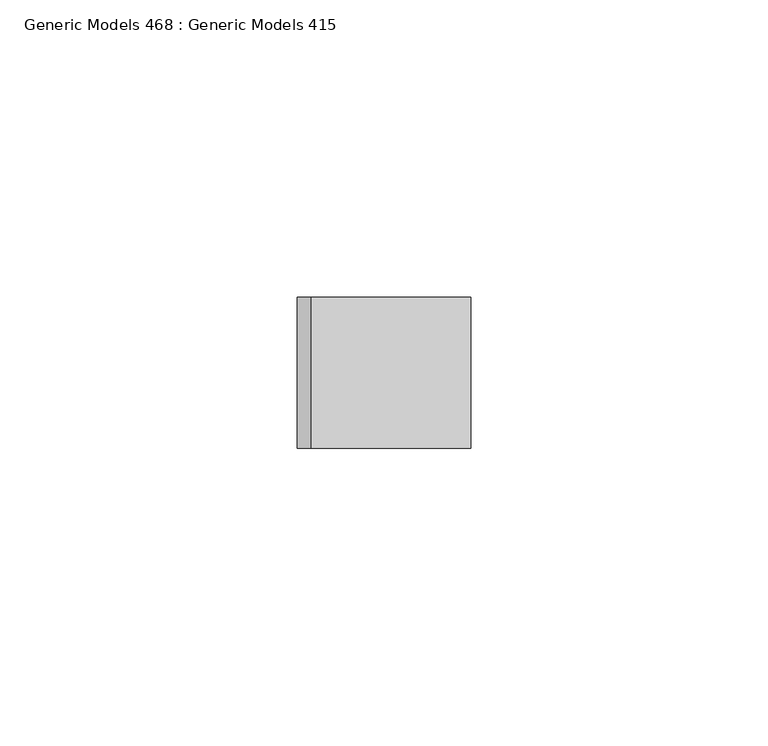
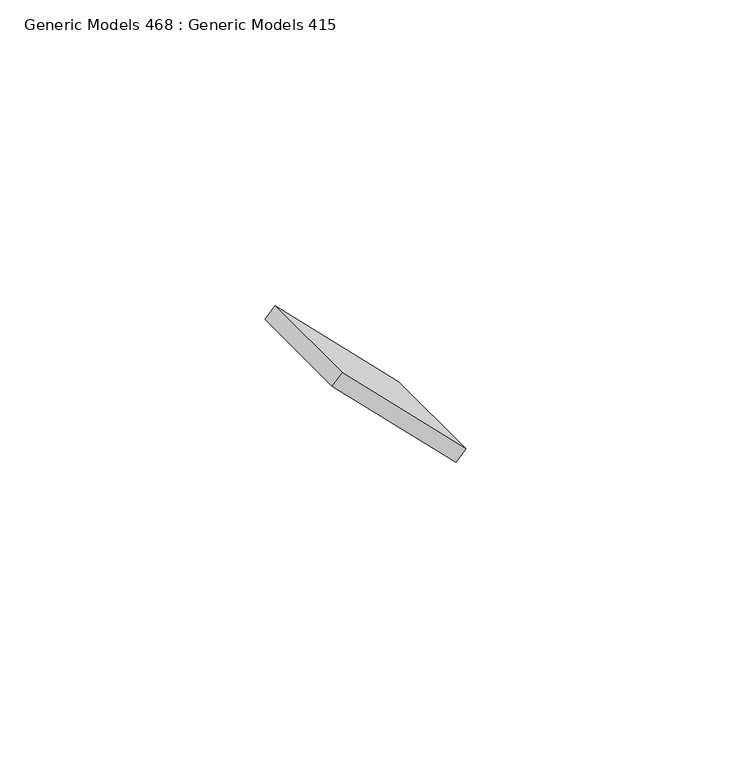
"""IFC4 building model written with IfcOpenShell, lengths in millimetres: proxy geometry, Generic Models 468 : Generic Models 415."""

from ifc_helpers import new_model, si_unit, frame, origin, place, context, project, spatial, polyline, outline, extrude, source, transform, mapped, element, save


def generic_models_468_generic_models_415_f77f82b4(model_context):
    return source(origin(), model_context, "Body", "SweptSolid", [
        extrude(outline(polyline([(0.0, -38.1), (0.0, 0.0), (25.4, 0.0), (25.4, -38.1), (0.0, -38.1)])), frame((-6869.8996186, -4475.9863946, 128226.0002957), z_axis=(0.7071067811864907, 0.0, 0.7071067811866044), x_axis=(0.0, -1.0, 0.0)), (0.0, 0.0, 1.0), 3.175),
    ])


if __name__ == "__main__":
    model = new_model("IFC4")
    model_context = context("Model", 3, world=origin())
    ifc_project = project(units=[si_unit("LENGTHUNIT", "METRE", prefix="MILLI")], contexts=[model_context])
    site = spatial("IfcSite", under=ifc_project)
    building = spatial("IfcBuilding", under=site)
    placement = place(None, origin())
    generic_models_468_generic_models_415_shape = generic_models_468_generic_models_415_f77f82b4(model_context)
    element("IfcBuildingElementProxy", 1, Name="Generic Models 468 : Generic Models 415", ObjectType="Generic Models 468 : Generic Models 415", at=placement, inside=building, context=model_context, shape_type="MappedRepresentation", body=[
        mapped(generic_models_468_generic_models_415_shape, transform((0.0, 0.0, 0.0), x_axis=(1.0, 0.0, 0.0), y_axis=(0.0, 1.0, 0.0), z_axis=(0.0, 0.0, 1.0))),
    ])
    save(model, "model.ifc")

# Revit data of these elements
# Element 1 (IfcBuildingElementProxy, "Generic Models 468 : Generic Models 415")
#   Materials on its faces: "_WELDED STEEL TABS FOR LOUVER ATTACHMENT"
# Materials
#   "_WELDED STEEL TABS FOR LOUVER ATTACHMENT": class "Metal", colour RGB 199 199 199, transparency 0, Description = "Structural steel 50ksi", Cost = 0
